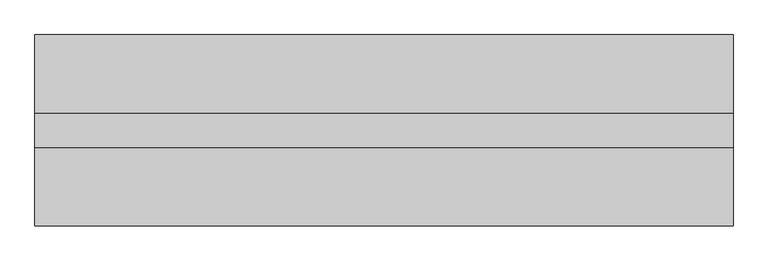
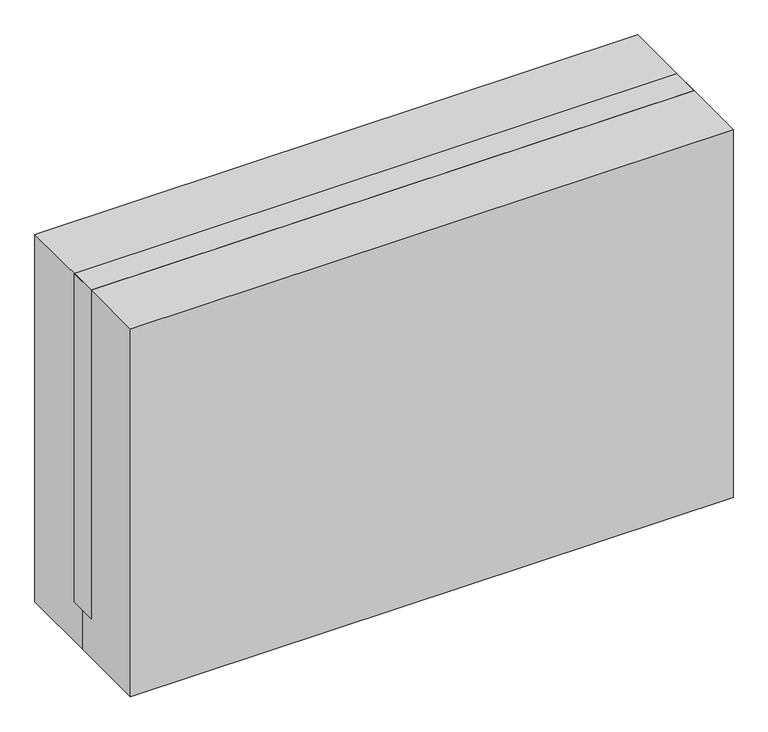
"""IFC4 building model written with IfcOpenShell, lengths in millimetres: proxy geometry, M0512 - Television, HDTV, Large Screen, 60in : M0512 - Television, HDTV, Large Screen, 60in."""

import ifcopenshell
import ifcopenshell.guid

model = None  # the IFC model being written
_history = None  # IfcOwnerHistory: only IFC2X3 demands one
_inside = {}  # id of a spatial element -> (the spatial element, [elements in it])
_under = {}  # id of a project, library or spatial element -> (it, [spatial elements below it])
_declared = {}  # id of a project -> (the project, [libraries it declares])
_typed = {}  # id of a type object -> (the type object, [elements of that type])
_made_of = {}  # id of a material, layer set ... -> (it, [elements and type objects made of it])


def new_model(schema):
    """Start an empty IFC model of exactly this schema.

    Asked for "IFC4X3", IfcOpenShell would pick the latest addendum, in which some entities
    have other attributes; the version numbers below select the first issue.
    IFC2X3 requires an IfcOwnerHistory on every rooted entity: one is made here for all.
    """
    global model, _history
    if schema == "IFC4X3":
        model = ifcopenshell.file(schema_version=(4, 3, 0, 0))
    else:
        model = ifcopenshell.file(schema=schema)
    _inside.clear()
    _under.clear()
    _declared.clear()
    _typed.clear()
    _made_of.clear()
    _history = None
    if model.schema == "IFC2X3":
        org = make("IfcOrganization", Name="unknown")
        user = make(
            "IfcPersonAndOrganization",
            ThePerson=make("IfcPerson", FamilyName="unknown"),
            TheOrganization=org,
        )
        app = make(
            "IfcApplication",
            ApplicationDeveloper=org,
            Version="unknown",
            ApplicationFullName="unknown",
            ApplicationIdentifier="unknown",
        )
        _history = make(
            "IfcOwnerHistory",
            OwningUser=user,
            OwningApplication=app,
            ChangeAction="ADDED",
            CreationDate=0,
        )
    return model


def make(cls, **values):
    """One entity of the class cls with the attributes given. An attribute that is None is left unset."""
    return model.create_entity(
        cls, **{name: value for name, value in values.items() if value is not None}
    )


def rooted(cls, **values):
    """An entity with a GlobalId (a new one), such as an element, a storey or a relation."""
    return make(cls, GlobalId=ifcopenshell.guid.new(), OwnerHistory=_history, **values)


def si_unit(unit_type, name, prefix=None):
    """IfcSIUnit, for example si_unit("LENGTHUNIT", "METRE", prefix="MILLI")."""
    return make("IfcSIUnit", UnitType=unit_type, Prefix=prefix, Name=name)


def assignment(units):
    """IfcUnitAssignment: the units of a project."""
    return None if units is None else make("IfcUnitAssignment", Units=units)


def point(xyz):
    """IfcCartesianPoint."""
    return None if xyz is None else make("IfcCartesianPoint", Coordinates=xyz)


def direction(xyz):
    """IfcDirection."""
    return None if xyz is None else make("IfcDirection", DirectionRatios=xyz)


def frame(location, z_axis=None, x_axis=None):
    """IfcAxis2Placement3D, a coordinate frame: its origin and axes. An axis left out is left unset."""
    return make(
        "IfcAxis2Placement3D",
        Location=point(location),
        Axis=direction(z_axis),
        RefDirection=direction(x_axis),
    )


def origin():
    """The frame at (0, 0, 0) with its axes left unset."""
    return frame((0.0, 0.0, 0.0))


def origin_with_axes():
    """The frame at (0, 0, 0) with the z axis (0, 0, 1) and the x axis (1, 0, 0) written out."""
    return frame((0.0, 0.0, 0.0), z_axis=(0.0, 0.0, 1.0), x_axis=(1.0, 0.0, 0.0))


def place(relative_to, where):
    """IfcLocalPlacement: puts the frame where relative to a parent placement (None: the world)."""
    return make(
        "IfcLocalPlacement", PlacementRelTo=relative_to, RelativePlacement=where
    )


def context(
    kind, dimensions, precision=None, world=None, true_north=None, identifier=None
):
    """IfcGeometricRepresentationContext, for example the 3D "Model" context."""
    return make(
        "IfcGeometricRepresentationContext",
        ContextIdentifier=identifier,
        ContextType=kind,
        CoordinateSpaceDimension=dimensions,
        Precision=precision,
        WorldCoordinateSystem=world,
        TrueNorth=true_north,
    )


def project(units=None, contexts=None):
    """IfcProject with its units and contexts."""
    return rooted(
        "IfcProject",
        Name="project",
        RepresentationContexts=contexts,
        UnitsInContext=assignment(units),
    )


def spatial(cls, under=None, at=None, **own):
    """A site, building, storey or space (cls), placed at a placement, below another one or the project."""
    s = rooted(cls, ObjectPlacement=at, **own)
    if under is not None:
        _under.setdefault(under.id(), (under, []))[1].append(s)
    return s


def polyline(points):
    """IfcPolyline through the points."""
    return make("IfcPolyline", Points=[point(p) for p in points])


def outline(outer, holes=None, kind="AREA"):
    """IfcArbitraryClosedProfileDef: a profile drawn as a closed curve; with holes, ...WithVoids."""
    if holes is None:
        return make("IfcArbitraryClosedProfileDef", ProfileType=kind, OuterCurve=outer)
    return make(
        "IfcArbitraryProfileDefWithVoids",
        ProfileType=kind,
        OuterCurve=outer,
        InnerCurves=holes,
    )


def extrude(swept, where, along, depth):
    """IfcExtrudedAreaSolid: the profile swept, set in the frame where, extruded along a direction by depth."""
    return make(
        "IfcExtrudedAreaSolid",
        SweptArea=swept,
        Position=where,
        ExtrudedDirection=direction(along),
        Depth=depth,
    )


def shape(context_of_items, identifier, shape_type, items):
    """IfcShapeRepresentation: the items that make up one representation, for example the "Body"."""
    return make(
        "IfcShapeRepresentation",
        ContextOfItems=context_of_items,
        RepresentationIdentifier=identifier,
        RepresentationType=shape_type,
        Items=items,
    )


def source(mapping_origin, context_of_items, identifier, shape_type, items):
    """IfcRepresentationMap: a shape defined once, which mapped items show again and again."""
    return make(
        "IfcRepresentationMap",
        MappingOrigin=mapping_origin,
        MappedRepresentation=shape(context_of_items, identifier, shape_type, items),
    )


def transform(
    local_origin,
    x_axis=None,
    y_axis=None,
    z_axis=None,
    scale=None,
    scale2=None,
    scale3=None,
    uniform=True,
):
    """IfcCartesianTransformationOperator3D, or its non-uniform kind. x_axis, y_axis, z_axis: its Axis1, 2, 3."""
    if uniform:
        return make(
            "IfcCartesianTransformationOperator3D",
            Axis1=direction(x_axis),
            Axis2=direction(y_axis),
            LocalOrigin=point(local_origin),
            Scale=scale,
            Axis3=direction(z_axis),
        )
    return make(
        "IfcCartesianTransformationOperator3DnonUniform",
        Axis1=direction(x_axis),
        Axis2=direction(y_axis),
        LocalOrigin=point(local_origin),
        Scale=scale,
        Axis3=direction(z_axis),
        Scale2=scale2,
        Scale3=scale3,
    )


def mapped(mapping_source, mapping_target):
    """IfcMappedItem: shows the shape of a source again, moved by a transform."""
    return make(
        "IfcMappedItem", MappingSource=mapping_source, MappingTarget=mapping_target
    )


def made_of(thing, what):
    """Note that an element or type object is made of a material, layer set ...; save() writes the relation."""
    if what is not None:
        _made_of.setdefault(what.id(), (what, []))[1].append(thing)
    return thing


def element(
    cls,
    number,
    at=None,
    inside=None,
    cuts=None,
    type_object=None,
    material=None,
    context=None,
    identifier="Body",
    shape_type=None,
    held_by="IfcProductDefinitionShape",
    body=None,
    shapes=None,
    **own,
):
    """One element of the class cls, such as IfcWall. Its Tag is "e" and its number.

    at: its placement. inside: the storey or other place that contains it. cuts: it is an
    opening in that element (IfcRelVoidsElement). A single representation is given by context,
    identifier, shape_type and body (its items); several are given by shapes. held_by: the class
    of the entity that holds the representations. save() writes the other relations.
    """
    e = rooted(cls, Tag="e%d" % number, ObjectPlacement=at, **own)
    if body is not None:
        shapes = [shape(context, identifier, shape_type, body)]
    if shapes is not None:
        e.Representation = make(held_by, Representations=shapes)
    if inside is not None:
        _inside.setdefault(inside.id(), (inside, []))[1].append(e)
    if cuts is not None:
        rooted(
            "IfcRelVoidsElement", RelatingBuildingElement=cuts, RelatedOpeningElement=e
        )
    if type_object is not None:
        _typed.setdefault(type_object.id(), (type_object, []))[1].append(e)
    return made_of(e, material)


def aggregate(whole, parts):
    """IfcRelAggregates: a whole, such as a stair, and the parts it consists of."""
    return rooted("IfcRelAggregates", RelatingObject=whole, RelatedObjects=parts)


def save(model, path):
    """Write the relations noted so far, then the file.

    IfcRelAggregates (storeys below a building ...), IfcRelContainedInSpatialStructure (elements
    in a storey), IfcRelDefinesByType, IfcRelAssociatesMaterial and IfcRelDeclares: one each for
    every whole, place, type object, material and project.
    """
    for whole, parts in _under.values():
        aggregate(whole, parts)
    for where, things in _inside.values():
        rooted(
            "IfcRelContainedInSpatialStructure",
            RelatedElements=things,
            RelatingStructure=where,
        )
    for kind, things in _typed.values():
        rooted("IfcRelDefinesByType", RelatedObjects=things, RelatingType=kind)
    for what, things in _made_of.values():
        rooted("IfcRelAssociatesMaterial", RelatedObjects=things, RelatingMaterial=what)
    for by, libraries in _declared.values():
        rooted("IfcRelDeclares", RelatingContext=by, RelatedDefinitions=libraries)
    model.write(path)


def specialty_equipment_e120b55a(model_context):
    return source(origin(), model_context, "Body", "SweptSolid", [
        extrude(outline(polyline([(1016.0, 787.4), (1016.0, -787.4), (107.95, -787.4), (107.95, 787.4), (1016.0, 787.4)]), holes=[polyline([(990.6, 762.0), (133.35, 762.0), (133.35, -762.0), (990.6, -762.0), (990.6, 762.0)])]), frame((0.0, -38.1, 0.0), z_axis=(0.0, 1.0, 0.0), x_axis=(0.0, 0.0, 1.0)), (0.0, 0.0, 1.0), 76.2),
        extrude(outline(polyline([(762.0, 12.7), (762.0, -38.1), (-762.0, -38.1), (-762.0, 12.7), (762.0, 12.7)])), frame((0.0, 0.0, 133.35), z_axis=(0.0, 0.0, 1.0), x_axis=(1.0, 0.0, 0.0)), (0.0, 0.0, 1.0), 857.25),
        extrude(outline(polyline([(-787.4, -215.9), (-787.4, 0.0), (-787.4, 215.9), (787.4, 215.9), (787.4, -215.9), (-787.4, -215.9)])), origin_with_axes(), (0.0, 0.0, 1.0), 1016.0),
    ])


if __name__ == "__main__":
    model = new_model("IFC4")
    model_context = context("Model", 3, world=origin())
    ifc_project = project(units=[si_unit("LENGTHUNIT", "METRE", prefix="MILLI")], contexts=[model_context])
    site = spatial("IfcSite", under=ifc_project)
    building = spatial("IfcBuilding", under=site)
    placement = place(None, origin())
    specialty_equipment_shape = specialty_equipment_e120b55a(model_context)
    element("IfcBuildingElementProxy", 1, Name="M0512 - Television, HDTV, Large Screen, 60in : M0512 - Television, HDTV, Large Screen, 60in", ObjectType="M0512 - Television, HDTV, Large Screen, 60in : M0512 - Television, HDTV, Large Screen, 60in", at=placement, inside=building, context=model_context, shape_type="MappedRepresentation", body=[
        mapped(specialty_equipment_shape, transform((0.0, 0.0, 0.0), x_axis=(1.0, 0.0, 0.0), y_axis=(0.0, 1.0, 0.0), z_axis=(0.0, 0.0, 1.0))),
    ])
    save(model, "model.ifc")

# Revit data of these elements
# Type "M0512 - Television, HDTV, Large Screen, 60in : M0512 - Television, HDTV, Large Screen, 60in"
#   Watts2 = "0"
#   Watts1 = "240"
#   Unit_Issue = "EA"
#   UTIL_6_Misc = "-"
#   UTIL_5_NonMedGas = "-"
#   UTIL_4_MiscGas = "-"
#   UTIL_3_MedGas = "-"
#   UTIL_2_Elec = "A"
#   UTIL_1_WaterDrain = "-"
#   Nomenclature = "Television, HDTV, Large Screen, 60\""
#   NSN = ""
#   Location [instance default] = ""
#   JSN = "M0512"
#   Fund_Source_VA = "-"
#   Fund_Source_Navy = "-"
#   Fund_Source_Army = "-"
#   Fund_Source_AF = "-"
#   ELEC_Volts2 = "0"
#   ELEC_Volts1 = "120"
#   ELEC_Phase2 = "0"
#   ELEC_Phase1 = "1"
#   ELEC_HertzSwitch = "0"
#   ELEC_HertzDependent = "-1"
#   ELEC_Hertz = "60"
#   ELEC_Amps2 = "0"
#   ELEC_Amps1 = "2"
#   DetailDescription = "A high definition (HDTV) multimedia, slim design, 60\"W to 65\"W color television. The TV will have a 16.9 wide screen aspect ratio with full HD 1080p resolution and HDMI connections. TV may be LED, Plasma or LCD. TV will include a stand."
#   CAT_VA = "C"
#   CAT_Navy = "C"
#   CAT_IHS = "-"
#   CAT_Army = "C"
#   CAT_AF = "C"
#   BTUperhour = "0"
#   Weight_IP = 88
#   DIM_Width_IP = 5' - 2"
#   DIM_Height_IP = 3' - 4"
#   DIM_Depth_IP = 1' - 5"
# Element 1 (IfcBuildingElementProxy, "M0512 - Television, HDTV, Large Screen, 60in : M0512 - Television, HDTV, Large Screen, 60in")
#   Materials on its faces: "EquipSpace"
# Materials
#   "EquipSpace": class "Unassigned", colour RGB 221 217 195, transparency 0.5
